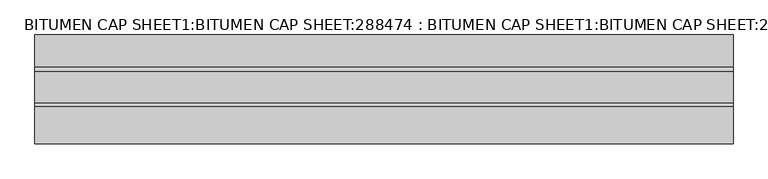
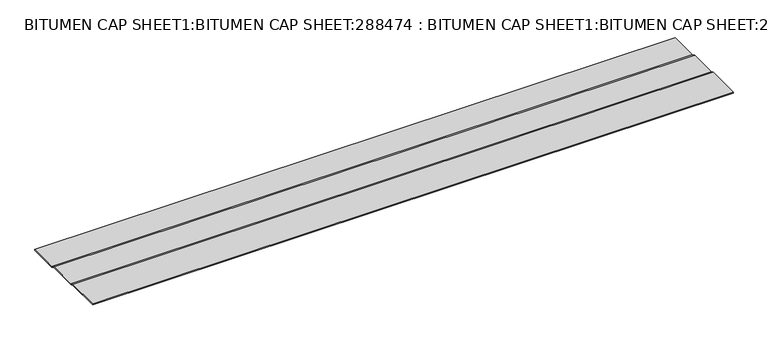
"""IFC4 building model written with IfcOpenShell, lengths in millimetres: proxy geometry, BITUMEN CAP SHEET1:BITUMEN CAP SHEET:288474 : BITUMEN CAP SHEET1:BITUMEN CAP SHEET:288474."""

from ifc_helpers import new_model, si_unit, frame, origin, place, context, project, spatial, polyline, outline, extrude, source, transform, mapped, element, save


def bitumen_cap_sheet1_bitumen_cap_sheet_288474_bitumen_cap_db1c2fb0(model_context):
    return source(origin(), model_context, "Body", "SweptSolid", [
        extrude(outline(polyline([(-4958.9432945, 40241.9330714), (-4958.9432945, 40238.7580714), (-5051.1079561, 40238.7580714), (-5063.5727747, 40244.0440809), (-5154.2869309, 40244.0440809), (-5164.0033174, 40248.3766459), (-5271.2145285, 40248.3766459), (-5271.2145285, 40251.5518755), (-5163.3280319, 40251.5518755), (-5153.6111304, 40247.2190809), (-5062.9273748, 40247.2190809), (-5050.4625561, 40241.9330714), (-4958.9432945, 40241.9330714)])), frame((17159.7769925, 0.0, 0.0), z_axis=(1.0, 0.0, 0.0), x_axis=(0.0, 1.0, 0.0)), (0.0, 0.0, 1.0), 2000.25),
    ])


if __name__ == "__main__":
    model = new_model("IFC4")
    model_context = context("Model", 3, world=origin())
    ifc_project = project(units=[si_unit("LENGTHUNIT", "METRE", prefix="MILLI")], contexts=[model_context])
    site = spatial("IfcSite", under=ifc_project)
    building = spatial("IfcBuilding", under=site)
    placement = place(None, origin())
    bitumen_cap_sheet1_bitumen_cap_sheet_288474_bitumen_cap_shape = bitumen_cap_sheet1_bitumen_cap_sheet_288474_bitumen_cap_db1c2fb0(model_context)
    element("IfcBuildingElementProxy", 1, Name="BITUMEN CAP SHEET1:BITUMEN CAP SHEET:288474 : BITUMEN CAP SHEET1:BITUMEN CAP SHEET:288474", ObjectType="BITUMEN CAP SHEET1:BITUMEN CAP SHEET:288474 : BITUMEN CAP SHEET1:BITUMEN CAP SHEET:288474", at=placement, inside=building, context=model_context, shape_type="MappedRepresentation", body=[
        mapped(bitumen_cap_sheet1_bitumen_cap_sheet_288474_bitumen_cap_shape, transform((0.0, 0.0, 0.0), x_axis=(1.0, 0.0, 0.0), y_axis=(0.0, 1.0, 0.0), z_axis=(0.0, 0.0, 1.0))),
    ])
    save(model, "model.ifc")

# Revit data of these elements
# Type "BITUMEN CAP SHEET1:BITUMEN CAP SHEET:288474 : BITUMEN CAP SHEET1:BITUMEN CAP SHEET:288474"
#   NameOverride = "BITUMEN CAP SHEET1:BITUMEN CAP SHEET:288474"
#   ObjectTypeOverride = "BITUMEN CAP SHEET1:BITUMEN CAP SHEET"
#   Reference = "BITUMEN CAP SHEET"
#   Category = "Generic Models"
#   Tag = "288474"
# Element 1 (IfcBuildingElementProxy, "BITUMEN CAP SHEET1:BITUMEN CAP SHEET:288474 : BITUMEN CAP SHEET1:BITUMEN CAP SHEET:288474")
#   Materials on its faces: "MODIFIED BITUMEN GRANULE SURFACED CAP SHEET"
# Materials
#   "MODIFIED BITUMEN GRANULE SURFACED CAP SHEET": class "Unassigned", colour RGB 85 85 127, transparency 0
